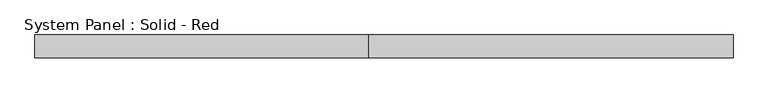
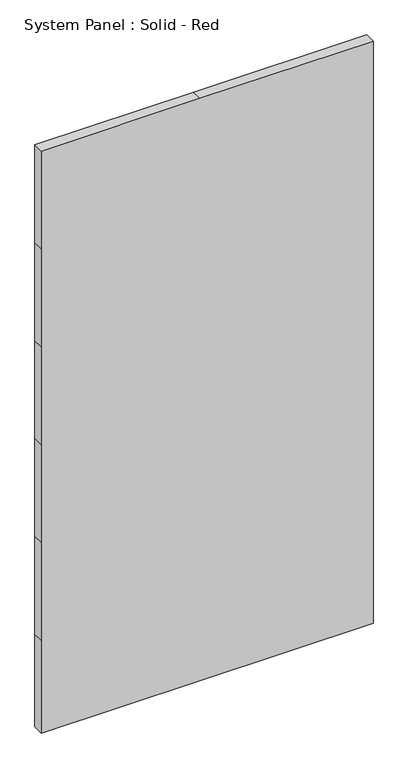
"""IFC4 building model written with IfcOpenShell, lengths in millimetres: plate geometry, System Panel : Solid - Red."""

import ifcopenshell
import ifcopenshell.guid

model = None  # the IFC model being written
_history = None  # IfcOwnerHistory: only IFC2X3 demands one
_inside = {}  # id of a spatial element -> (the spatial element, [elements in it])
_under = {}  # id of a project, library or spatial element -> (it, [spatial elements below it])
_declared = {}  # id of a project -> (the project, [libraries it declares])
_typed = {}  # id of a type object -> (the type object, [elements of that type])
_made_of = {}  # id of a material, layer set ... -> (it, [elements and type objects made of it])


def new_model(schema):
    """Start an empty IFC model of exactly this schema.

    Asked for "IFC4X3", IfcOpenShell would pick the latest addendum, in which some entities
    have other attributes; the version numbers below select the first issue.
    IFC2X3 requires an IfcOwnerHistory on every rooted entity: one is made here for all.
    """
    global model, _history
    if schema == "IFC4X3":
        model = ifcopenshell.file(schema_version=(4, 3, 0, 0))
    else:
        model = ifcopenshell.file(schema=schema)
    _inside.clear()
    _under.clear()
    _declared.clear()
    _typed.clear()
    _made_of.clear()
    _history = None
    if model.schema == "IFC2X3":
        org = make("IfcOrganization", Name="unknown")
        user = make(
            "IfcPersonAndOrganization",
            ThePerson=make("IfcPerson", FamilyName="unknown"),
            TheOrganization=org,
        )
        app = make(
            "IfcApplication",
            ApplicationDeveloper=org,
            Version="unknown",
            ApplicationFullName="unknown",
            ApplicationIdentifier="unknown",
        )
        _history = make(
            "IfcOwnerHistory",
            OwningUser=user,
            OwningApplication=app,
            ChangeAction="ADDED",
            CreationDate=0,
        )
    return model


def make(cls, **values):
    """One entity of the class cls with the attributes given. An attribute that is None is left unset."""
    return model.create_entity(
        cls, **{name: value for name, value in values.items() if value is not None}
    )


def rooted(cls, **values):
    """An entity with a GlobalId (a new one), such as an element, a storey or a relation."""
    return make(cls, GlobalId=ifcopenshell.guid.new(), OwnerHistory=_history, **values)


def si_unit(unit_type, name, prefix=None):
    """IfcSIUnit, for example si_unit("LENGTHUNIT", "METRE", prefix="MILLI")."""
    return make("IfcSIUnit", UnitType=unit_type, Prefix=prefix, Name=name)


def assignment(units):
    """IfcUnitAssignment: the units of a project."""
    return None if units is None else make("IfcUnitAssignment", Units=units)


def point(xyz):
    """IfcCartesianPoint."""
    return None if xyz is None else make("IfcCartesianPoint", Coordinates=xyz)


def direction(xyz):
    """IfcDirection."""
    return None if xyz is None else make("IfcDirection", DirectionRatios=xyz)


def frame(location, z_axis=None, x_axis=None):
    """IfcAxis2Placement3D, a coordinate frame: its origin and axes. An axis left out is left unset."""
    return make(
        "IfcAxis2Placement3D",
        Location=point(location),
        Axis=direction(z_axis),
        RefDirection=direction(x_axis),
    )


def origin():
    """The frame at (0, 0, 0) with its axes left unset."""
    return frame((0.0, 0.0, 0.0))


def place(relative_to, where):
    """IfcLocalPlacement: puts the frame where relative to a parent placement (None: the world)."""
    return make(
        "IfcLocalPlacement", PlacementRelTo=relative_to, RelativePlacement=where
    )


def context(
    kind, dimensions, precision=None, world=None, true_north=None, identifier=None
):
    """IfcGeometricRepresentationContext, for example the 3D "Model" context."""
    return make(
        "IfcGeometricRepresentationContext",
        ContextIdentifier=identifier,
        ContextType=kind,
        CoordinateSpaceDimension=dimensions,
        Precision=precision,
        WorldCoordinateSystem=world,
        TrueNorth=true_north,
    )


def project(units=None, contexts=None):
    """IfcProject with its units and contexts."""
    return rooted(
        "IfcProject",
        Name="project",
        RepresentationContexts=contexts,
        UnitsInContext=assignment(units),
    )


def spatial(cls, under=None, at=None, **own):
    """A site, building, storey or space (cls), placed at a placement, below another one or the project."""
    s = rooted(cls, ObjectPlacement=at, **own)
    if under is not None:
        _under.setdefault(under.id(), (under, []))[1].append(s)
    return s


def polyline(points):
    """IfcPolyline through the points."""
    return make("IfcPolyline", Points=[point(p) for p in points])


def outline(outer, holes=None, kind="AREA"):
    """IfcArbitraryClosedProfileDef: a profile drawn as a closed curve; with holes, ...WithVoids."""
    if holes is None:
        return make("IfcArbitraryClosedProfileDef", ProfileType=kind, OuterCurve=outer)
    return make(
        "IfcArbitraryProfileDefWithVoids",
        ProfileType=kind,
        OuterCurve=outer,
        InnerCurves=holes,
    )


def extrude(swept, where, along, depth):
    """IfcExtrudedAreaSolid: the profile swept, set in the frame where, extruded along a direction by depth."""
    return make(
        "IfcExtrudedAreaSolid",
        SweptArea=swept,
        Position=where,
        ExtrudedDirection=direction(along),
        Depth=depth,
    )


def shape(context_of_items, identifier, shape_type, items):
    """IfcShapeRepresentation: the items that make up one representation, for example the "Body"."""
    return make(
        "IfcShapeRepresentation",
        ContextOfItems=context_of_items,
        RepresentationIdentifier=identifier,
        RepresentationType=shape_type,
        Items=items,
    )


def source(mapping_origin, context_of_items, identifier, shape_type, items):
    """IfcRepresentationMap: a shape defined once, which mapped items show again and again."""
    return make(
        "IfcRepresentationMap",
        MappingOrigin=mapping_origin,
        MappedRepresentation=shape(context_of_items, identifier, shape_type, items),
    )


def transform(
    local_origin,
    x_axis=None,
    y_axis=None,
    z_axis=None,
    scale=None,
    scale2=None,
    scale3=None,
    uniform=True,
):
    """IfcCartesianTransformationOperator3D, or its non-uniform kind. x_axis, y_axis, z_axis: its Axis1, 2, 3."""
    if uniform:
        return make(
            "IfcCartesianTransformationOperator3D",
            Axis1=direction(x_axis),
            Axis2=direction(y_axis),
            LocalOrigin=point(local_origin),
            Scale=scale,
            Axis3=direction(z_axis),
        )
    return make(
        "IfcCartesianTransformationOperator3DnonUniform",
        Axis1=direction(x_axis),
        Axis2=direction(y_axis),
        LocalOrigin=point(local_origin),
        Scale=scale,
        Axis3=direction(z_axis),
        Scale2=scale2,
        Scale3=scale3,
    )


def mapped(mapping_source, mapping_target):
    """IfcMappedItem: shows the shape of a source again, moved by a transform."""
    return make(
        "IfcMappedItem", MappingSource=mapping_source, MappingTarget=mapping_target
    )


def made_of(thing, what):
    """Note that an element or type object is made of a material, layer set ...; save() writes the relation."""
    if what is not None:
        _made_of.setdefault(what.id(), (what, []))[1].append(thing)
    return thing


def element(
    cls,
    number,
    at=None,
    inside=None,
    cuts=None,
    type_object=None,
    material=None,
    context=None,
    identifier="Body",
    shape_type=None,
    held_by="IfcProductDefinitionShape",
    body=None,
    shapes=None,
    **own,
):
    """One element of the class cls, such as IfcWall. Its Tag is "e" and its number.

    at: its placement. inside: the storey or other place that contains it. cuts: it is an
    opening in that element (IfcRelVoidsElement). A single representation is given by context,
    identifier, shape_type and body (its items); several are given by shapes. held_by: the class
    of the entity that holds the representations. save() writes the other relations.
    """
    e = rooted(cls, Tag="e%d" % number, ObjectPlacement=at, **own)
    if body is not None:
        shapes = [shape(context, identifier, shape_type, body)]
    if shapes is not None:
        e.Representation = make(held_by, Representations=shapes)
    if inside is not None:
        _inside.setdefault(inside.id(), (inside, []))[1].append(e)
    if cuts is not None:
        rooted(
            "IfcRelVoidsElement", RelatingBuildingElement=cuts, RelatedOpeningElement=e
        )
    if type_object is not None:
        _typed.setdefault(type_object.id(), (type_object, []))[1].append(e)
    return made_of(e, material)


def aggregate(whole, parts):
    """IfcRelAggregates: a whole, such as a stair, and the parts it consists of."""
    return rooted("IfcRelAggregates", RelatingObject=whole, RelatedObjects=parts)


def save(model, path):
    """Write the relations noted so far, then the file.

    IfcRelAggregates (storeys below a building ...), IfcRelContainedInSpatialStructure (elements
    in a storey), IfcRelDefinesByType, IfcRelAssociatesMaterial and IfcRelDeclares: one each for
    every whole, place, type object, material and project.
    """
    for whole, parts in _under.values():
        aggregate(whole, parts)
    for where, things in _inside.values():
        rooted(
            "IfcRelContainedInSpatialStructure",
            RelatedElements=things,
            RelatingStructure=where,
        )
    for kind, things in _typed.values():
        rooted("IfcRelDefinesByType", RelatedObjects=things, RelatingType=kind)
    for what, things in _made_of.values():
        rooted("IfcRelAssociatesMaterial", RelatedObjects=things, RelatingMaterial=what)
    for by, libraries in _declared.values():
        rooted("IfcRelDeclares", RelatingContext=by, RelatedDefinitions=libraries)
    model.write(path)


def system_panel_solid_red_e56ed630(model_context):
    return source(origin(), model_context, "Body", "SweptSolid", [
        extrude(outline(polyline([(0.0, -977.9), (0.0, -43.3916667), (0.0, 977.9), (577.85, 977.9), (1187.45, 977.9), (1797.05, 977.9), (2406.65, 977.9), (3016.25, 977.9), (3625.85, 977.9), (3625.85, -43.3916667), (3625.85, -977.9), (3016.25, -977.9), (2406.65, -977.9), (1797.05, -977.9), (1187.45, -977.9), (577.85, -977.9), (0.0, -977.9)])), frame((0.0, -44.45, 0.0), z_axis=(0.0, 1.0, 0.0), x_axis=(0.0, 0.0, 1.0)), (0.0, 0.0, 1.0), 63.5),
    ])


if __name__ == "__main__":
    model = new_model("IFC4")
    model_context = context("Model", 3, world=origin())
    ifc_project = project(units=[si_unit("LENGTHUNIT", "METRE", prefix="MILLI")], contexts=[model_context])
    site = spatial("IfcSite", under=ifc_project)
    building = spatial("IfcBuilding", under=site)
    placement = place(None, origin())
    system_panel_solid_red_shape = system_panel_solid_red_e56ed630(model_context)
    element("IfcPlate", 1, ObjectType="System Panel : Solid - Red", at=placement, inside=building, context=model_context, shape_type="MappedRepresentation", body=[
        mapped(system_panel_solid_red_shape, transform((0.0, 0.0, 0.0), x_axis=(1.0, 0.0, 0.0), y_axis=(0.0, 1.0, 0.0), z_axis=(0.0, 0.0, 1.0))),
    ])
    save(model, "model.ifc")

# Revit data of these elements
# Project information
#   SR Document GUID = "d36f5d78-752a-40d6-a009-b379f065f3eb"
# Element 1 (IfcPlate, "System Panel : Solid - Red")
#   Materials on its faces: "Red Panel"
# Materials
#   "Red Panel": class "Unassigned", colour RGB 255 0 0, transparency 0
